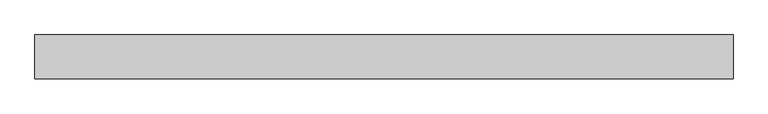
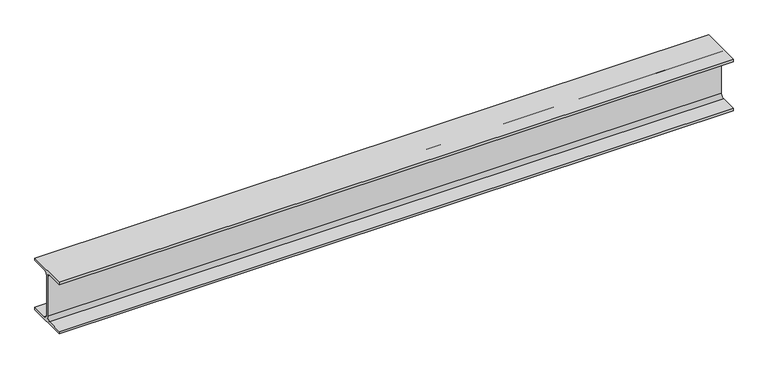
"""IFC4 building model written with IfcOpenShell, lengths in millimetres: beam geometry, 0912_Steel Framing_H-KSD3502 : H_SB_ASB_H-194x150x6x9."""

from ifc_helpers import new_model, si_unit, point, frame, frame_2d, origin, place, context, project, spatial, polyline, circle_curve, trimmed, segment, composite_curve, outline, extrude, source, transform, mapped, element, save


def beam_00fabe47(model_context):
    return source(origin(), model_context, "Body", "SweptSolid", [
        extrude(outline(composite_curve([segment(polyline([(-75.0, -88.0), (-16.0, -88.0)]), True, "CONTINUOUS"), segment(trimmed(circle_curve(frame_2d((-16.0, -75.0)), 13.0), [point((-16.0, -88.0))], [point((-3.0, -75.0))], True, "CARTESIAN"), True, "CONTINUOUS"), segment(polyline([(-3.0, -75.0), (-3.0, 75.0)]), True, "CONTINUOUS"), segment(trimmed(circle_curve(frame_2d((-16.0, 75.0)), 13.0), [point((-3.0, 75.0))], [point((-16.0, 88.0))], True, "CARTESIAN"), True, "CONTINUOUS"), segment(polyline([(-16.0, 88.0), (-75.0, 88.0), (-75.0, 97.0), (75.0, 97.0), (75.0, 88.0), (16.0, 88.0)]), True, "CONTINUOUS"), segment(trimmed(circle_curve(frame_2d((16.0, 75.0)), 13.0), [point((16.0, 88.0))], [point((3.0, 75.0))], True, "CARTESIAN"), True, "CONTINUOUS"), segment(polyline([(3.0, 75.0), (3.0, -75.0)]), True, "CONTINUOUS"), segment(trimmed(circle_curve(frame_2d((16.0, -75.0)), 13.0), [point((3.0, -75.0))], [point((16.0, -88.0))], True, "CARTESIAN"), True, "CONTINUOUS"), segment(polyline([(16.0, -88.0), (75.0, -88.0), (75.0, -97.0), (-75.0, -97.0), (-75.0, -88.0)]), True, "CONTINUOUS")], self_intersect=False)), frame((-1068.0314701, 0.0, 0.0), z_axis=(1.0, 0.0, 0.0), x_axis=(0.0, 1.0, 0.0)), (0.0, 0.0, 1.0), 2394.2341721),
    ])


if __name__ == "__main__":
    model = new_model("IFC4")
    model_context = context("Model", 3, world=origin())
    ifc_project = project(units=[si_unit("LENGTHUNIT", "METRE", prefix="MILLI")], contexts=[model_context])
    site = spatial("IfcSite", under=ifc_project)
    building = spatial("IfcBuilding", under=site)
    placement = place(None, origin())
    beam_shape = beam_00fabe47(model_context)
    element("IfcBeam", 1, ObjectType="0912_Steel Framing_H-KSD3502 : H_SB_ASB_H-194x150x6x9", at=placement, inside=building, context=model_context, shape_type="MappedRepresentation", body=[
        mapped(beam_shape, transform((0.0, 0.0, 0.0), x_axis=(1.0, 0.0, 0.0), y_axis=(0.0, 1.0, 0.0), z_axis=(0.0, 0.0, 1.0))),
    ])
    save(model, "model.ifc")

# Revit data of these elements
# Type "0912_Steel Framing_H-KSD3502 : H_SB_ASB_H-194x150x6x9"
#   H_WM Code_1 = "S01AA002-00001 | Main Steel Structure Fabrication Work | Shelter/Building | Medium Steel - Standard (90KG/M>Weight≥30KG/M) | Material: (   )"
#   H_WM Code_2 = "S03AA028-00001 | Main Steel Structure Erection Work | Shelter/Building | Medium Steel (90KG/M>Weight≥30KG/M) | Material: (   )"
#   H_WM Code_3 = "S01AA010-00001 | Main Steel Structure Fabrication Work | Shelter/Building | Steel Painting/Coating | for Non-Fireproofed Steel Surface, Surface Preparation, Primer, Second & Final Coat | Material: (   )"
#   H_Q'ty Cal Type Tag = "SB-Q2"
#   Width = 15.0 cm
#   Web Thickness = 0.6 cm
#   Web Fillet = 1.3 cm
#   Warping Constant = 43316.0 cm⁶
#   W = 0
#   Torsional Moment of Inertia = 8.622 cm⁴
#   Section Area = 39.01 cm²
#   Plastic Modulus weak axis = 104.0 cm³
#   Plastic Modulus strong axis = 309.0 cm³
#   Perimeter = 0.95 m²/m
#   Nominal Weight = 30.60 kgf/m
#   Moment of Inertia weak axis = 507.00 cm⁴
#   Moment of Inertia strong axis = 2690.00 cm⁴
#   Height = 19.4 cm
#   Flange Thickness = 0.9 cm
#   Elastic Modulus weak axis = 67.6 cm³
#   Elastic Modulus strong axis = 277.0 cm³
#   Centroid Vertical = 9.7 cm
#   Centroid Horizontal = 7.5 cm
#   Ix = 26900000
#   Length [instance default] = 1.5240 m
#   Zx = 309000
#   b = 0.1500 m
#   h = 0.1940 m
#   r = 0.0130 m
#   s = 0.0060 m
#   t = 0.0090 m
#   A = 0.003901 m²
#   Structural Material [instance default] = Steel, 45-345
#   Assembly Code = ""
# Element 1 (IfcBeam, "0912_Steel Framing_H-KSD3502 : H_SB_ASB_H-194x150x6x9")
#   Structural Material = none
# Materials
#   "Steel, 45-345": class "Metal", colour RGB 189 187 185, transparency 0, Description = "Steel 345 MPa", Cost = 0
